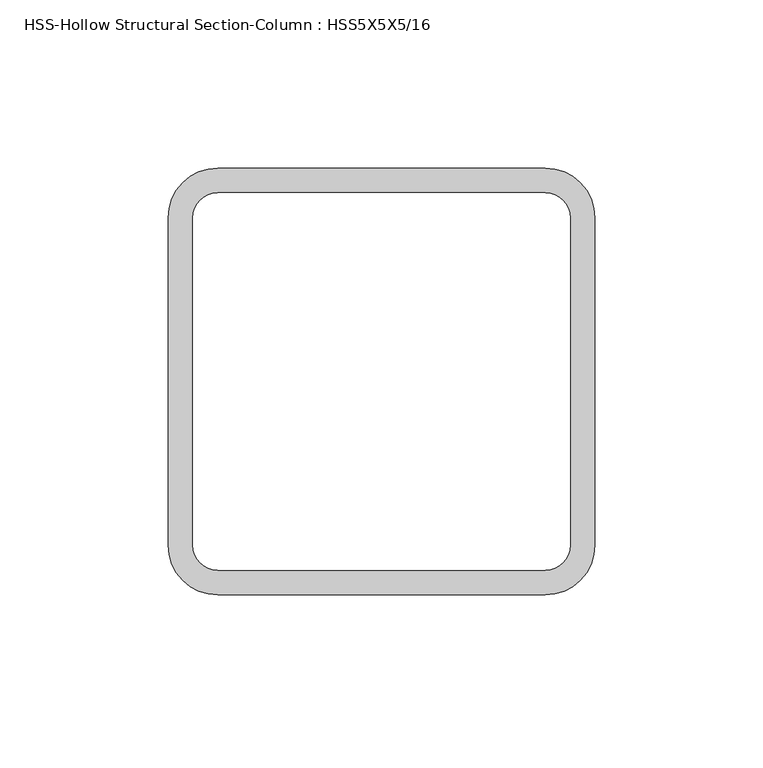
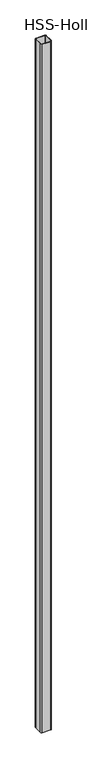
"""IFC4 building model written with IfcOpenShell, lengths in millimetres: column geometry, HSS-Hollow Structural Section-Column : HSS5X5X5/16."""

from ifc_helpers import new_model, si_unit, point, frame, frame_2d, origin, place, context, project, spatial, polyline, circle_curve, trimmed, segment, composite_curve, outline, extrude, source, transform, mapped, element, save


def hss_hollow_structural_section_column_hss5x5x5_16_1dd65b46(model_context):
    return source(origin(), model_context, "Body", "SweptSolid", [
        extrude(outline(composite_curve([segment(trimmed(circle_curve(frame_2d((48.7172, 48.7172)), 14.7828), [point((48.7172, 63.5))], [point((63.5, 48.7172))], False, "CARTESIAN"), True, "CONTINUOUS"), segment(polyline([(63.5, 48.7172), (63.5, -48.7172)]), True, "CONTINUOUS"), segment(trimmed(circle_curve(frame_2d((48.7172, -48.7172)), 14.7828), [point((63.5, -48.7172))], [point((48.7172, -63.5))], False, "CARTESIAN"), True, "CONTINUOUS"), segment(polyline([(48.7172, -63.5), (-48.7172, -63.5)]), True, "CONTINUOUS"), segment(trimmed(circle_curve(frame_2d((-48.7172, -48.7172)), 14.7828), [point((-48.7172, -63.5))], [point((-63.5, -48.7172))], False, "CARTESIAN"), True, "CONTINUOUS"), segment(polyline([(-63.5, -48.7172), (-63.5, 48.7172)]), True, "CONTINUOUS"), segment(trimmed(circle_curve(frame_2d((-48.7172, 48.7172)), 14.7828), [point((-63.5, 48.7172))], [point((-48.7172, 63.5))], False, "CARTESIAN"), True, "CONTINUOUS"), segment(polyline([(-48.7172, 63.5), (48.7172, 63.5)]), True, "CONTINUOUS")], self_intersect=False), holes=[composite_curve([segment(polyline([(48.7172, 56.1086), (-48.7172, 56.1086)]), True, "CONTINUOUS"), segment(trimmed(circle_curve(frame_2d((-48.7172, 48.7172)), 7.3914), [point((-48.7172, 56.1086))], [point((-56.1086, 48.7172))], True, "CARTESIAN"), True, "CONTINUOUS"), segment(polyline([(-56.1086, 48.7172), (-56.1086, -48.7172)]), True, "CONTINUOUS"), segment(trimmed(circle_curve(frame_2d((-48.7172, -48.7172)), 7.3914), [point((-56.1086, -48.7172))], [point((-48.7172, -56.1086))], True, "CARTESIAN"), True, "CONTINUOUS"), segment(polyline([(-48.7172, -56.1086), (48.7172, -56.1086)]), True, "CONTINUOUS"), segment(trimmed(circle_curve(frame_2d((48.7172, -48.7172)), 7.3914), [point((48.7172, -56.1086))], [point((56.1086, -48.7172))], True, "CARTESIAN"), True, "CONTINUOUS"), segment(polyline([(56.1086, -48.7172), (56.1086, 48.7172)]), True, "CONTINUOUS"), segment(trimmed(circle_curve(frame_2d((48.7172, 48.7172)), 7.3914), [point((56.1086, 48.7172))], [point((48.7172, 56.1086))], True, "CARTESIAN"), True, "CONTINUOUS")], self_intersect=False)]), frame((0.0, 0.0, 16408.4), z_axis=(0.0, 0.0, 1.0), x_axis=(1.0, 0.0, 0.0)), (0.0, 0.0, 1.0), 8534.4),
    ])


if __name__ == "__main__":
    model = new_model("IFC4")
    model_context = context("Model", 3, world=origin())
    ifc_project = project(units=[si_unit("LENGTHUNIT", "METRE", prefix="MILLI")], contexts=[model_context])
    site = spatial("IfcSite", under=ifc_project)
    building = spatial("IfcBuilding", under=site)
    placement = place(None, origin())
    hss_hollow_structural_section_column_hss5x5x5_16_shape = hss_hollow_structural_section_column_hss5x5x5_16_1dd65b46(model_context)
    element("IfcColumn", 1, ObjectType="HSS-Hollow Structural Section-Column : HSS5X5X5/16", at=placement, inside=building, context=model_context, shape_type="MappedRepresentation", body=[
        mapped(hss_hollow_structural_section_column_hss5x5x5_16_shape, transform((0.0, 0.0, 0.0), x_axis=(1.0, 0.0, 0.0), y_axis=(0.0, 1.0, 0.0), z_axis=(0.0, 0.0, 1.0))),
    ])
    save(model, "model.ifc")

# Revit data of these elements
# Type "HSS-Hollow Structural Section-Column : HSS5X5X5/16"
#   Assembly Code = "B10"
#   Shape = "Square"
#   W = 19
#   Ht = 0' - 5"
#   b = 0' - 5"
#   kr = 0' - 0.582"
#   t = 0' - 0.291"
#   A = 0.0365278 SF
#   Structural Material [instance default] = Steel ASTM A500, Grade B, Rectangular and Square
# Element 1 (IfcColumn, "HSS-Hollow Structural Section-Column : HSS5X5X5/16")
#   Materials on its faces: "Steel ASTM A500, Grade B, Rectangular and Square"
# Materials
#   "Steel ASTM A500, Grade B, Rectangular and Square": class "Metal", colour RGB 199 199 199, transparency 0, Description = "Carbon steel", Cost = 0
